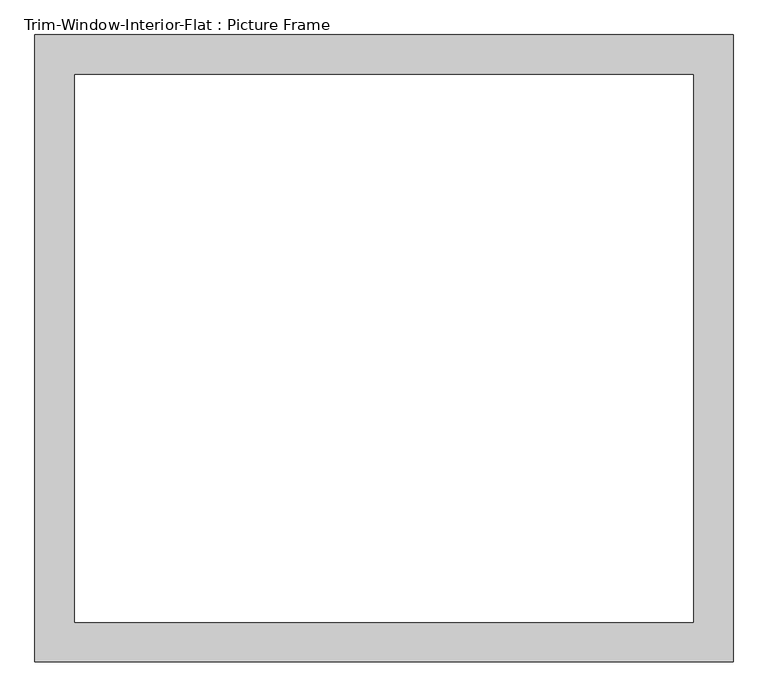
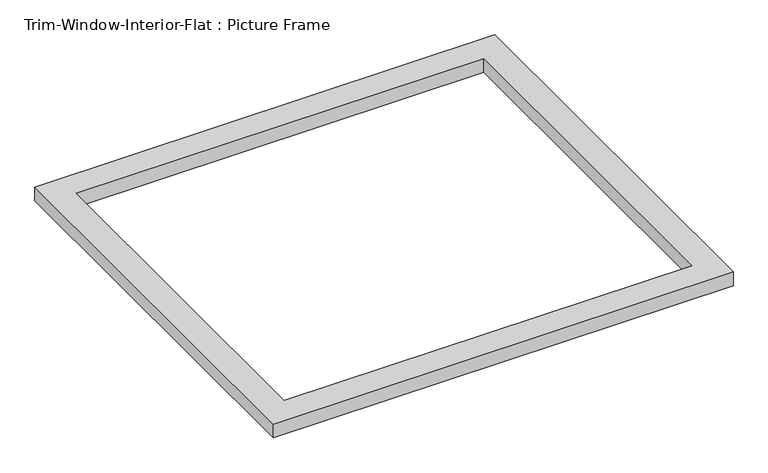
"""IFC4 building model written with IfcOpenShell, lengths in millimetres: proxy geometry, Trim-Window-Interior-Flat : Picture Frame."""

from ifc_helpers import new_model, si_unit, origin, origin_with_axes, place, context, project, spatial, polyline, outline, extrude, source, transform, mapped, element, save


def trim_window_interior_flat_picture_frame_c9ba522f(model_context):
    return source(origin(), model_context, "Body", "SweptSolid", [
        extrude(outline(polyline([(501.65, 44.45), (501.65, -857.25), (-501.65, -857.25), (-501.65, 44.45), (501.65, 44.45)]), holes=[polyline([(444.5, -12.7), (-444.5, -12.7), (-444.5, -800.1), (444.5, -800.1), (444.5, -12.7)])]), origin_with_axes(), (0.0, 0.0, 1.0), 31.75),
    ])


if __name__ == "__main__":
    model = new_model("IFC4")
    model_context = context("Model", 3, world=origin())
    ifc_project = project(units=[si_unit("LENGTHUNIT", "METRE", prefix="MILLI")], contexts=[model_context])
    site = spatial("IfcSite", under=ifc_project)
    building = spatial("IfcBuilding", under=site)
    placement = place(None, origin())
    trim_window_interior_flat_picture_frame_shape = trim_window_interior_flat_picture_frame_c9ba522f(model_context)
    element("IfcBuildingElementProxy", 1, Name="Trim-Window-Interior-Flat : Picture Frame", ObjectType="Trim-Window-Interior-Flat : Picture Frame", at=placement, inside=building, context=model_context, shape_type="MappedRepresentation", body=[
        mapped(trim_window_interior_flat_picture_frame_shape, transform((0.0, 0.0, 0.0), x_axis=(1.0, 0.0, 0.0), y_axis=(0.0, 1.0, 0.0), z_axis=(0.0, 0.0, 1.0))),
    ])
    save(model, "model.ifc")

# Revit data of these elements
# Type "Trim-Window-Interior-Flat : Picture Frame"
#   Trim Thickness_Picture Frame = 0' - 1 1/4"
#   Trim Width = 0' - 2 1/4"
#   Trim Thickness_with Sill = 0' - 0 3/4"
#   Sill Thickness = 0' - 1 1/4"
#   Opening Width [instance default] = 2' - 0"
#   Opening Height [instance default] = 3' - 0"
#   Default Elevation = 4' - 0"
#   Sill = no
#   Picture Frame = yes
#   Trim Material [instance default] = none
# Element 1 (IfcBuildingElementProxy, "Trim-Window-Interior-Flat : Picture Frame")
#   Opening Width = 3' - 0"
#   Opening Height = 2' - 8"
#   Trim Material = Maple - Semigloss(Rotated)
#   Materials on its faces: "Maple - Semigloss(Rotated)"
# Materials
#   "Maple - Semigloss(Rotated)": class "Wood", colour RGB 196 161 118, transparency 0, Description = "Acer Saccharum", Cost = 0
